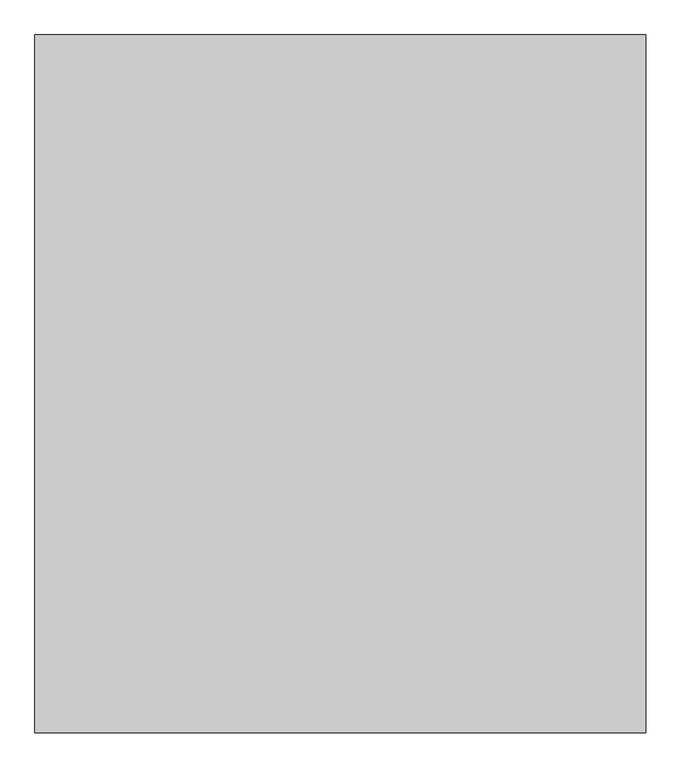
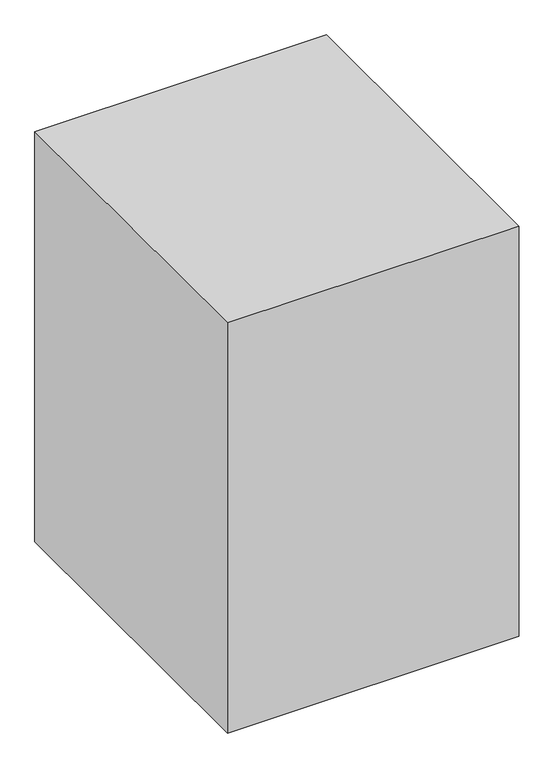
"""IFC4 building model written with IfcOpenShell, lengths in millimetres: proxy geometry, Space Planning Box_hec : Space Planning Box_hec."""

from ifc_helpers import new_model, si_unit, origin, origin_with_axes, place, context, project, spatial, polyline, outline, extrude, source, transform, mapped, element, save


def generic_models_7d267c0d(model_context):
    return source(origin(), model_context, "Body", "SweptSolid", [
        extrude(outline(polyline([(1750.0, 2000.0), (1750.0, -2000.0), (-1750.0, -2000.0), (-1750.0, 2000.0), (1750.0, 2000.0)])), origin_with_axes(), (0.0, 0.0, 1.0), 5200.0),
    ])


if __name__ == "__main__":
    model = new_model("IFC4")
    model_context = context("Model", 3, world=origin())
    ifc_project = project(units=[si_unit("LENGTHUNIT", "METRE", prefix="MILLI")], contexts=[model_context])
    site = spatial("IfcSite", under=ifc_project)
    building = spatial("IfcBuilding", under=site)
    placement = place(None, origin())
    generic_models_shape = generic_models_7d267c0d(model_context)
    element("IfcBuildingElementProxy", 1, Name="Space Planning Box_hec : Space Planning Box_hec", ObjectType="Space Planning Box_hec : Space Planning Box_hec", at=placement, inside=building, context=model_context, shape_type="MappedRepresentation", body=[
        mapped(generic_models_shape, transform((0.0, 0.0, 0.0), x_axis=(1.0, 0.0, 0.0), y_axis=(0.0, 1.0, 0.0), z_axis=(0.0, 0.0, 1.0))),
    ])
    save(model, "model.ifc")

# Revit data of these elements
# Type "Space Planning Box_hec : Space Planning Box_hec"
#   Type Comments = "..."
#   Room Name [instance default] = "?"
#   Interior Finish [instance default] = ""
#   Exterior Finish [instance default] = ""
#   Department [instance default] = ""
#   Assembly Code = "..."
#   ceiling height [instance default] = 0
#   Width [instance default] = 1524 mm
#   Program Area [instance default] = 0.00 m²
#   Length [instance default] = 1524 mm
#   Height [instance default] = 1524 mm
#   Area [instance default] = 2.32258 m²
#   Fill Color [instance default] = Cyan
#   Default Elevation = 0
# Element 1 (IfcBuildingElementProxy, "Space Planning Box_hec : Space Planning Box_hec")
#   Room Name = "Pantry"
#   Interior Finish = "IW1..N/A,,WB2..N/A,,FL6..N/A,,CL4..N/A"
#   Exterior Finish = "RF1..N/A,,EW1..N/A"
#   Department = "AR"
#   ceiling height = 2700
#   Width = 3500 mm
#   Program Area = 14.00 m²
#   Length = 4000 mm
#   Height = 5200 mm
#   Area = 14.00 m²
#   Materials on its faces: "Cyan"
# Materials
#   "Cyan": class "Generic", colour RGB 0 255 255, transparency 0.2, Cost = 0
